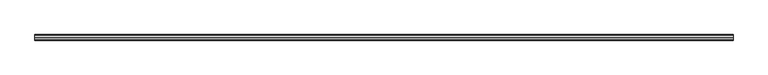
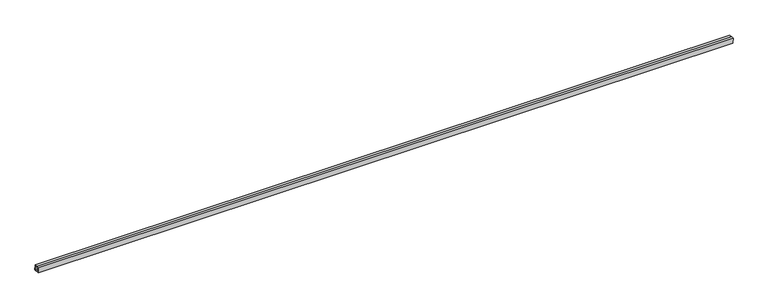
"""IFC4 building model written with IfcOpenShell, lengths in millimetres: proxy geometry, Inner panel:Inner panel:1:Inner panel:1 : Inner panel:Inner panel:300324:2:Inner panel:1:Inner panel:1 : Inner panel:Inner panel:300324:2 : Inner panel:Inner panel:1:Inner panel:1 : Inner panel:Inner panel:300324:300043:22 : Inner panel:Inner panel:1:Inner panel:1 : Inner panel:Inner panel:300324:2:Inner panel:1:Inner panel:1 : Inner panel:Inner panel:300324:2 : Inner panel:Inner panel:1:Inner panel:1 : Inner panel:Inner panel:300324:300043:308120."""

from ifc_helpers import new_model, si_unit, frame, origin, place, context, project, spatial, polyline, outline, extrude, source, transform, mapped, element, save


def generic_models_bdf7f818(model_context):
    return source(origin(), model_context, "Body", "SweptSolid", [
        extrude(outline(polyline([(-579091.9810065, 3946.0946172), (-579073.7405833, 3946.8546348), (-579072.1544596, 3908.7876647), (-579110.2214297, 3907.201541), (-579111.8075534, 3945.268511), (-579093.5671303, 3946.0285287), (-579093.4679975, 3943.649343), (-579109.3292351, 3942.9884581), (-579107.9413768, 3909.6798593), (-579074.632778, 3911.0677176), (-579076.0206362, 3944.3763164), (-579091.8818738, 3943.7154315), (-579091.9810065, 3946.0946172)])), frame((591883.8891713, 0.0, 0.0), z_axis=(1.0, 0.0, 0.0), x_axis=(0.0, 1.0, 0.0)), (0.0, 0.0, 1.0), 4914.8975526),
    ])


if __name__ == "__main__":
    model = new_model("IFC4")
    model_context = context("Model", 3, world=origin())
    ifc_project = project(units=[si_unit("LENGTHUNIT", "METRE", prefix="MILLI")], contexts=[model_context])
    site = spatial("IfcSite", under=ifc_project)
    building = spatial("IfcBuilding", under=site)
    placement = place(None, origin())
    generic_models_shape = generic_models_bdf7f818(model_context)
    element("IfcBuildingElementProxy", 1, Name="Inner panel:Inner panel:1:Inner panel:1 : Inner panel:Inner panel:300324:2:Inner panel:1:Inner panel:1 : Inner panel:Inner panel:300324:2 : Inner panel:Inner panel:1:Inner panel:1 : Inner panel:Inner panel:300324:300043:22 : Inner panel:Inner panel:1:Inner panel:1 : Inner panel:Inner panel:300324:2:Inner panel:1:Inner panel:1 : Inner panel:Inner panel:300324:2 : Inner panel:Inner panel:1:Inner panel:1 : Inner panel:Inner panel:300324:300043:308120", ObjectType="Inner panel:Inner panel:1:Inner panel:1 : Inner panel:Inner panel:300324:2:Inner panel:1:Inner panel:1 : Inner panel:Inner panel:300324:2 : Inner panel:Inner panel:1:Inner panel:1 : Inner panel:Inner panel:300324:300043:22 : Inner panel:Inner panel:1:Inner panel:1 : Inner panel:Inner panel:300324:2:Inner panel:1:Inner panel:1 : Inner panel:Inner panel:300324:2 : Inner panel:Inner panel:1:Inner panel:1 : Inner panel:Inner panel:300324:300043:308120", at=placement, inside=building, context=model_context, shape_type="MappedRepresentation", body=[
        mapped(generic_models_shape, transform((0.0, 0.0, 0.0), x_axis=(1.0, 0.0, 0.0), y_axis=(0.0, 1.0, 0.0), z_axis=(0.0, 0.0, 1.0))),
    ])
    save(model, "model.ifc")

# Revit data of these elements
# Type "Inner panel:Inner panel:1:Inner panel:1 : Inner panel:Inner panel:300324:2:Inner panel:1:Inner panel:1 : Inner panel:Inner panel:300324:2 : Inner panel:Inner panel:1:Inner panel:1 : Inner panel:Inner panel:300324:300043:22 : Inner panel:Inner panel:1:Inner panel:1 : Inner panel:Inner panel:300324:2:Inner panel:1:Inner panel:1 : Inner panel:Inner panel:300324:2 : Inner panel:Inner panel:1:Inner panel:1 : Inner panel:Inner panel:300324:300043:308120"
#   NameOverride = "Inner panel:Inner panel:1:Inner panel:1 : Inner panel:Inner panel:300324:2:Inner panel:1:Inner panel:1 : Inner panel:Inner panel:300324:2 : Inner panel:Inner panel:1:Inner panel:1 : Inner panel:Inner panel:300324:300043:308120"
#   ObjectTypeOverride = "Inner panel:1:Inner panel:1 : Inner panel:Inner panel:300324:2 : Inner panel:Inner panel:1:Inner panel:1 : Inner panel:Inner panel:300324:300043"
#   Reference = "Inner panel"
#   Tag = "308120"
# Element 1 (IfcBuildingElementProxy, "Inner panel:Inner panel:1:Inner panel:1 : Inner panel:Inner panel:300324:2:Inner panel:1:Inner panel:1 : Inner panel:Inner panel:300324:2 : Inner panel:Inner panel:1:Inner panel:1 : Inner panel:Inner panel:300324:300043:22 : Inner panel:Inner panel:1:Inner panel:1 : Inner panel:Inner panel:300324:2:Inner panel:1:Inner panel:1 : Inner panel:Inner panel:300324:2 : Inner panel:Inner panel:1:Inner panel:1 : Inner panel:Inner panel:300324:300043:308120")
#   Materials on its faces: "1 1/2\" X 1 1/2\" SPLIT-SEAM SQUARE TUBING (~24\" CANTILEVER FROM C.L. OF GLULAM)"
# Materials
#   "1 1/2\" X 1 1/2\" SPLIT-SEAM SQUARE TUBING (~24\" CANTILEVER FROM C.L. OF GLULAM)": class "Unassigned", colour RGB 202 201 200, transparency 0, Cost = 0
